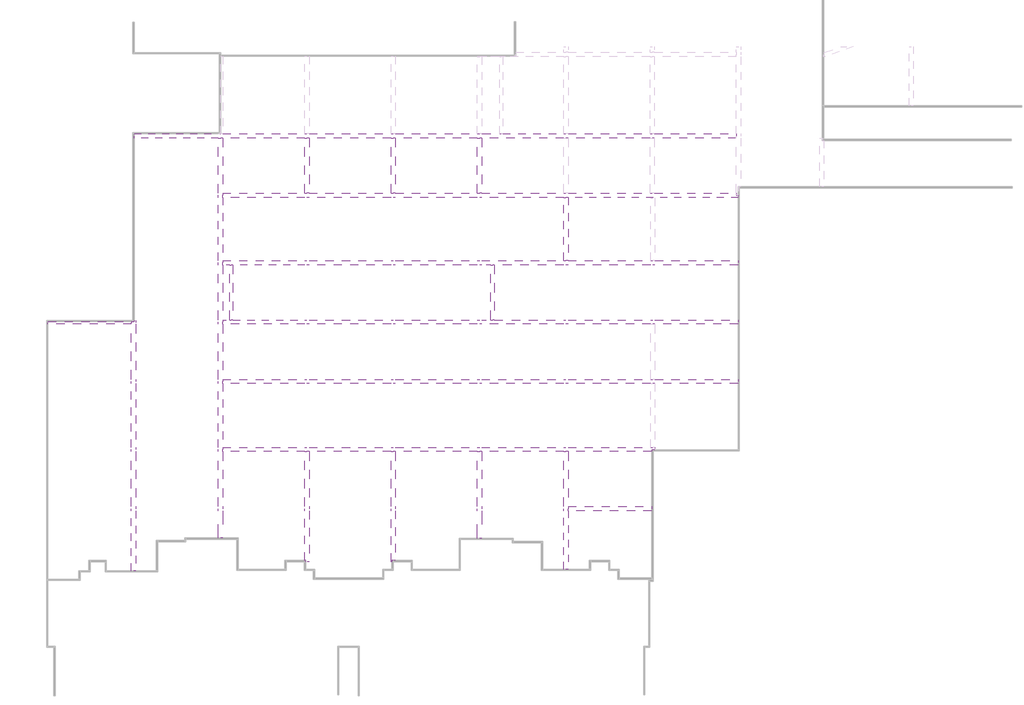
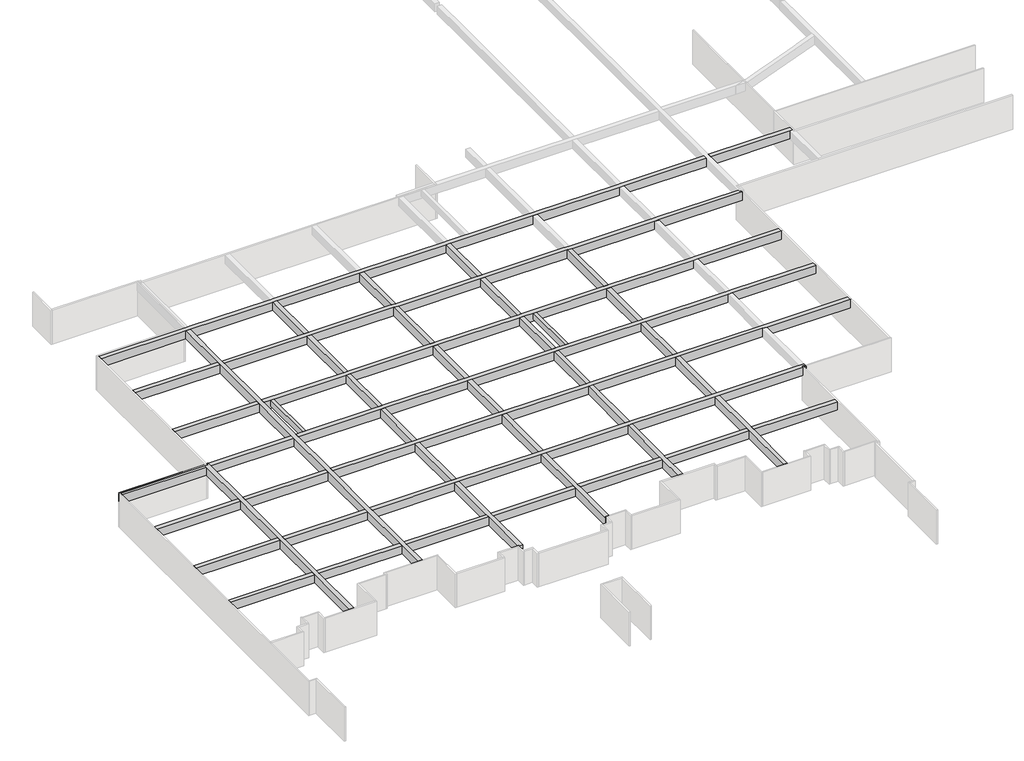
# One storey, part 7 of 14: 20 beams.
"""IFC4 building model written with IfcOpenShell, lengths in millimetres."""

from ifc_helpers import new_model, si_unit, frame, origin, place, context, project, spatial, polyline, outline, extrude, faceted_brep, element, save

model = new_model("IFC4")

# Units and contexts
model_context = context("Model", 3, world=origin())
ifc_project = project(units=[si_unit("LENGTHUNIT", "METRE", prefix="MILLI")], contexts=[model_context])

# Site, building, storey
site = spatial("IfcSite", under=ifc_project)
building = spatial("IfcBuilding", under=site)
storey = spatial("IfcBuildingStorey", under=building, Name="户型图", Elevation=0.0)

# Beams
placement = place(None, origin())
element("IfcBeam", 1, ObjectType="混凝土 - 矩形梁 : KL_beam", at=placement, inside=storey, context=model_context, shape_type="Brep", body=[
    faceted_brep([(-586071.2602569, -192842.8565135, 3300.0), (-586071.2602569, -193242.8565135, 3300.0), (-578267.6529954, -193242.8565135, 3300.0), (-577867.6529954, -193242.8565135, 3300.0), (-570267.6529954, -193242.8565135, 3300.0), (-569867.6529954, -193242.8565135, 3300.0), (-562267.6529954, -193242.8565135, 3300.0), (-561867.6529954, -193242.8565135, 3300.0), (-554267.6529954, -193242.8565135, 3300.0), (-553867.6529954, -193242.8565135, 3300.0), (-546267.6529954, -193242.8565135, 3300.0), (-545867.6529954, -193242.8565135, 3300.0), (-538267.6529954, -193242.8565135, 3300.0), (-537867.6529954, -193242.8565135, 3300.0), (-530267.6529954, -193242.8565135, 3300.0), (-530267.6529954, -192842.8565135, 3300.0), (-537867.6529954, -192842.8565135, 3300.0), (-538267.6529954, -192842.8565135, 3300.0), (-545867.6529954, -192842.8565135, 3300.0), (-546267.6529954, -192842.8565135, 3300.0), (-551917.6529953, -192842.8565135, 3300.0), (-552217.6529953, -192842.8565135, 3300.0), (-553867.6529954, -192842.8565135, 3300.0), (-554267.6529954, -192842.8565135, 3300.0), (-561867.6529954, -192842.8565135, 3300.0), (-562267.6529954, -192842.8565135, 3300.0), (-569867.6529954, -192842.8565135, 3300.0), (-570267.6529954, -192842.8565135, 3300.0), (-577867.6529954, -192842.8565135, 3300.0), (-578267.6529954, -192842.8565135, 3300.0), (-586071.2602569, -193242.8565135, 2500.0), (-578267.6529954, -193242.8565135, 2500.0), (-577867.6529954, -193242.8565135, 2500.0), (-570267.6529954, -193242.8565135, 2500.0), (-569867.6529954, -193242.8565135, 2500.0), (-562267.6529954, -193242.8565135, 2500.0), (-561867.6529954, -193242.8565135, 2500.0), (-554267.6529954, -193242.8565135, 2500.0), (-553867.6529954, -193242.8565135, 2500.0), (-546267.6529954, -193242.8565135, 2500.0), (-545867.6529954, -193242.8565135, 2500.0), (-538267.6529954, -193242.8565135, 2500.0), (-537867.6529954, -193242.8565135, 2500.0), (-530267.6529954, -193242.8565135, 2500.0), (-586071.2602569, -192842.8565135, 2500.0), (-578267.6529954, -192842.8565135, 2500.0), (-577867.6529954, -192842.8565135, 2500.0), (-570267.6529954, -192842.8565135, 2500.0), (-569867.6529954, -192842.8565135, 2500.0), (-562267.6529954, -192842.8565135, 2500.0), (-561867.6529954, -192842.8565135, 2500.0), (-554267.6529954, -192842.8565135, 2500.0), (-553867.6529954, -192842.8565135, 2500.0), (-546267.6529954, -192842.8565135, 2500.0), (-545867.6529954, -192842.8565135, 2500.0), (-538267.6529954, -192842.8565135, 2500.0), (-537867.6529954, -192842.8565135, 2500.0), (-530267.6529954, -192842.8565135, 2500.0)], [[[0, 1, 2, 3, 4, 5, 6, 7, 8, 9, 10, 11, 12, 13, 14, 15, 16, 17, 18, 19, 20, 21, 22, 23, 24, 25, 26, 27, 28, 29]], [[1, 30, 31, 32, 33, 34, 35, 36, 37, 38, 39, 40, 41, 42, 43, 14, 13, 12, 11, 10, 9, 8, 7, 6, 5, 4, 3, 2]], [[30, 44, 45, 46, 47, 48, 49, 50, 51, 52, 53, 54, 55, 56, 57, 43, 42, 41, 40, 39, 38, 37, 36, 35, 34, 33, 32, 31]], [[44, 0, 29, 28, 27, 26, 25, 24, 23, 22, 21, 20, 19, 18, 17, 16, 15, 57, 56, 55, 54, 53, 52, 51, 50, 49, 48, 47, 46, 45]], [[1, 0, 44, 30]], [[15, 14, 43, 57]]]),
    faceted_brep([(-522315.6671501, -192842.8565135, 3300.0), (-522315.6671501, -193242.8565135, 3300.0), (-522315.6671501, -193242.8565135, 2500.0), (-522315.6671501, -192842.8565135, 2500.0), (-529867.6529954, -193242.8565135, 3300.0), (-529867.6529954, -192842.8565135, 3300.0), (-529867.6529954, -192842.8565135, 2500.0), (-529867.6529954, -193242.8565135, 2500.0), (-522567.6529953, -193242.8565135, 3300.0), (-522567.6529953, -193242.8565135, 2500.0)], [[[0, 1, 2, 3]], [[4, 5, 6, 7]], [[1, 0, 5, 4, 8]], [[2, 1, 8, 4, 7, 9]], [[3, 2, 9, 7, 6]], [[0, 3, 6, 5]]]),
])
element("IfcBeam", 2, ObjectType="混凝土 - 矩形梁 : KL_beam", at=placement, inside=storey, context=model_context, shape_type="Brep", body=[
    faceted_brep([(-578267.6529954, -230304.5164481, 3300.0), (-577867.6529954, -230304.5164481, 3300.0), (-577867.6529954, -227792.8565135, 3300.0), (-577867.6529954, -227392.8565135, 3300.0), (-577867.6529954, -222292.8565135, 3300.0), (-577867.6529954, -221892.8565135, 3300.0), (-577867.6529954, -215992.8565135, 3300.0), (-577867.6529954, -215592.8565135, 3300.0), (-577867.6529954, -210492.8565135, 3300.0), (-577867.6529954, -210092.8565135, 3300.0), (-577867.6529954, -204992.8565135, 3300.0), (-577867.6529954, -204592.8565135, 3300.0), (-577867.6529954, -198734.4327531, 3300.0), (-577867.6529954, -198334.4327531, 3300.0), (-577867.6529954, -193242.8565135, 3300.0), (-578267.6529954, -193242.8565135, 3300.0), (-578267.6529954, -198334.4327531, 3300.0), (-578267.6529954, -198734.4327531, 3300.0), (-578267.6529954, -204592.8565135, 3300.0), (-578267.6529954, -204992.8565135, 3300.0), (-578267.6529954, -210092.8565135, 3300.0), (-578267.6529954, -210492.8565135, 3300.0), (-578267.6529954, -215592.8565135, 3300.0), (-578267.6529954, -215992.8565135, 3300.0), (-578267.6529954, -221892.8565135, 3300.0), (-578267.6529954, -222292.8565135, 3300.0), (-578267.6529954, -227392.8565135, 3300.0), (-578267.6529954, -227792.8565135, 3300.0), (-578267.6529954, -230304.5164481, 2500.0), (-578267.6529954, -193242.8565135, 2500.0), (-578267.6529954, -198334.4327531, 2500.0), (-578267.6529954, -198734.4327531, 2500.0), (-578267.6529954, -204592.8565135, 2500.0), (-578267.6529954, -204992.8565135, 2500.0), (-578267.6529954, -210092.8565135, 2500.0), (-578267.6529954, -210492.8565135, 2500.0), (-578267.6529954, -215592.8565135, 2500.0), (-578267.6529954, -215992.8565135, 2500.0), (-578267.6529954, -221892.8565135, 2500.0), (-578267.6529954, -222292.8565135, 2500.0), (-578267.6529954, -227392.8565135, 2500.0), (-578267.6529954, -227792.8565135, 2500.0), (-577867.6529954, -230304.5164481, 2500.0), (-577867.6529954, -193242.8565135, 2500.0), (-577867.6529954, -198334.4327531, 2500.0), (-577867.6529954, -198734.4327531, 2500.0), (-577867.6529954, -204592.8565135, 2500.0), (-577867.6529954, -204992.8565135, 2500.0), (-577867.6529954, -210092.8565135, 2500.0), (-577867.6529954, -210492.8565135, 2500.0), (-577867.6529954, -215592.8565135, 2500.0), (-577867.6529954, -215992.8565135, 2500.0), (-577867.6529954, -221892.8565135, 2500.0), (-577867.6529954, -222292.8565135, 2500.0), (-577867.6529954, -227392.8565135, 2500.0), (-577867.6529954, -227792.8565135, 2500.0)], [[[0, 1, 2, 3, 4, 5, 6, 7, 8, 9, 10, 11, 12, 13, 14, 15, 16, 17, 18, 19, 20, 21, 22, 23, 24, 25, 26, 27]], [[28, 0, 27, 26, 25, 24, 23, 22, 21, 20, 19, 18, 17, 16, 15, 29, 30, 31, 32, 33, 34, 35, 36, 37, 38, 39, 40, 41]], [[42, 28, 41, 40, 39, 38, 37, 36, 35, 34, 33, 32, 31, 30, 29, 43, 44, 45, 46, 47, 48, 49, 50, 51, 52, 53, 54, 55]], [[1, 42, 55, 54, 53, 52, 51, 50, 49, 48, 47, 46, 45, 44, 43, 14, 13, 12, 11, 10, 9, 8, 7, 6, 5, 4, 3, 2]], [[1, 0, 28, 42]], [[15, 14, 43, 29]]]),
])
element("IfcBeam", 3, ObjectType="混凝土 - 矩形梁 : KL_beam", at=placement, inside=storey, context=model_context, shape_type="Brep", body=[
    faceted_brep([(-586071.2602569, -210252.8565135, 3300.0), (-586191.2602569, -210252.8565135, 3300.0), (-586331.2602569, -210252.8565135, 3300.0), (-586331.2602569, -210492.8565135, 3300.0), (-586331.2602569, -215592.8565135, 3300.0), (-586331.2602569, -215992.8565135, 3300.0), (-586331.2602569, -221892.8565135, 3300.0), (-586331.2602569, -222292.8565135, 3300.0), (-586331.2602569, -227392.8565135, 3300.0), (-586331.2602569, -227792.8565135, 3300.0), (-586331.2602569, -233343.599968, 3300.0), (-585931.2602569, -233343.599968, 3300.0), (-585931.2602569, -227792.8565135, 3300.0), (-585931.2602569, -227392.8565135, 3300.0), (-585931.2602569, -222292.8565135, 3300.0), (-585931.2602569, -221892.8565135, 3300.0), (-585931.2602569, -215992.8565135, 3300.0), (-585931.2602569, -215592.8565135, 3300.0), (-585931.2602569, -210492.8565135, 3300.0), (-585931.2602569, -210132.8565135, 3300.0), (-586071.2602569, -210132.8565135, 3300.0), (-586331.2602569, -210252.8565135, 2500.0), (-586331.2602569, -210492.8565135, 2500.0), (-586331.2602569, -215592.8565135, 2500.0), (-586331.2602569, -215992.8565135, 2500.0), (-586331.2602569, -221892.8565135, 2500.0), (-586331.2602569, -222292.8565135, 2500.0), (-586331.2602569, -227392.8565135, 2500.0), (-586331.2602569, -227792.8565135, 2500.0), (-586331.2602569, -233343.599968, 2500.0), (-586071.2602569, -210252.8565135, 2500.0), (-586071.2602569, -210132.8565135, 2500.0), (-585931.2602569, -210132.8565135, 2500.0), (-585931.2602569, -210492.8565135, 2500.0), (-585931.2602569, -215592.8565135, 2500.0), (-585931.2602569, -215992.8565135, 2500.0), (-585931.2602569, -221892.8565135, 2500.0), (-585931.2602569, -222292.8565135, 2500.0), (-585931.2602569, -227392.8565135, 2500.0), (-585931.2602569, -227792.8565135, 2500.0), (-585931.2602569, -233343.599968, 2500.0)], [[[0, 1, 2, 3, 4, 5, 6, 7, 8, 9, 10, 11, 12, 13, 14, 15, 16, 17, 18, 19, 20]], [[2, 21, 22, 23, 24, 25, 26, 27, 28, 29, 10, 9, 8, 7, 6, 5, 4, 3]], [[21, 30, 31, 32, 33, 34, 35, 36, 37, 38, 39, 40, 29, 28, 27, 26, 25, 24, 23, 22]], [[32, 19, 18, 17, 16, 15, 14, 13, 12, 11, 40, 39, 38, 37, 36, 35, 34, 33]], [[19, 32, 31, 20]], [[0, 30, 21, 2, 1]], [[11, 10, 29, 40]], [[30, 0, 20, 31]]]),
])
element("IfcBeam", 4, ObjectType="混凝土 - 矩形梁 : KL_beam", at=placement, inside=storey, context=model_context, shape_type="SweptSolid", body=[
    extrude(outline(polyline([(-594071.2602569, -210492.8565135), (-594071.2602569, -210252.8565135), (-586331.2602569, -210252.8565135), (-586331.2602569, -210492.8565135), (-594071.2602569, -210492.8565135)])), frame((0.0, 0.0, 2500.0), z_axis=(0.0, 0.0, 1.0), x_axis=(1.0, 0.0, 0.0)), (0.0, 0.0, 1.0), 800.0),
    extrude(outline(polyline([(-585931.2602569, -210092.8565135), (-585931.2602569, -210132.8565135), (-586071.2602569, -210132.8565135), (-586071.2602569, -210092.8565135), (-585931.2602569, -210092.8565135)])), frame((0.0, 0.0, 2500.0), z_axis=(0.0, 0.0, 1.0), x_axis=(1.0, 0.0, 0.0)), (0.0, 0.0, 1.0), 800.0),
    extrude(outline(polyline([(-594191.2602569, -210132.8565135), (-594191.2602569, -210092.8565135), (-586191.2602569, -210092.8565135), (-586191.2602569, -210132.8565135), (-594191.2602569, -210132.8565135)])), frame((0.0, 0.0, 2500.0), z_axis=(0.0, 0.0, 1.0), x_axis=(1.0, 0.0, 0.0)), (0.0, 0.0, 1.0), 800.0),
])
element("IfcBeam", 5, ObjectType="混凝土 - 矩形梁 : KL_beam", at=placement, inside=storey, context=model_context, shape_type="Brep", body=[
    faceted_brep([(-585931.2602569, -210092.8565135, 3300.0), (-585931.2602569, -210132.8565135, 3300.0), (-585931.2602569, -210492.8565135, 3300.0), (-578267.6529954, -210492.8565135, 3300.0), (-578267.6529954, -210092.8565135, 3300.0), (-585931.2602569, -210492.8565135, 2500.0), (-578267.6529954, -210492.8565135, 2500.0), (-585931.2602569, -210132.8565135, 2500.0), (-585931.2602569, -210092.8565135, 2500.0), (-578267.6529954, -210092.8565135, 2500.0)], [[[0, 1, 2, 3, 4]], [[2, 5, 6, 3]], [[5, 7, 8, 9, 6]], [[8, 0, 4, 9]], [[5, 2, 1, 0, 8, 7]], [[4, 3, 6, 9]]]),
    faceted_brep([(-530117.7352575, -210092.8565135, 3300.0), (-530117.7352575, -210492.8565135, 3300.0), (-530117.7352575, -210492.8565135, 2500.0), (-530117.7352575, -210092.8565135, 2500.0), (-577867.6529954, -210492.8565135, 3300.0), (-577867.6529954, -210092.8565135, 3300.0), (-577867.6529954, -210092.8565135, 2500.0), (-577867.6529954, -210492.8565135, 2500.0), (-537831.2602569, -210092.8565135, 3300.0), (-538231.2602569, -210092.8565135, 3300.0), (-545867.6529954, -210092.8565135, 3300.0), (-546267.6529954, -210092.8565135, 3300.0), (-552717.6529953, -210092.8565135, 3300.0), (-553017.6529953, -210092.8565135, 3300.0), (-553867.6529954, -210092.8565135, 3300.0), (-554267.6529954, -210092.8565135, 3300.0), (-561867.6529954, -210092.8565135, 3300.0), (-562267.6529954, -210092.8565135, 3300.0), (-569867.6529954, -210092.8565135, 3300.0), (-570267.6529954, -210092.8565135, 3300.0), (-576917.6529953, -210092.8565135, 3300.0), (-577217.6529953, -210092.8565135, 3300.0), (-570267.6529954, -210492.8565135, 3300.0), (-569867.6529954, -210492.8565135, 3300.0), (-562267.6529954, -210492.8565135, 3300.0), (-561867.6529954, -210492.8565135, 3300.0), (-554267.6529954, -210492.8565135, 3300.0), (-553867.6529954, -210492.8565135, 3300.0), (-546267.6529954, -210492.8565135, 3300.0), (-545867.6529954, -210492.8565135, 3300.0), (-538231.2602569, -210492.8565135, 3300.0), (-537831.2602569, -210492.8565135, 3300.0), (-570267.6529954, -210492.8565135, 2500.0), (-569867.6529954, -210492.8565135, 2500.0), (-562267.6529954, -210492.8565135, 2500.0), (-561867.6529954, -210492.8565135, 2500.0), (-554267.6529954, -210492.8565135, 2500.0), (-553867.6529954, -210492.8565135, 2500.0), (-546267.6529954, -210492.8565135, 2500.0), (-545867.6529954, -210492.8565135, 2500.0), (-538231.2602569, -210492.8565135, 2500.0), (-537831.2602569, -210492.8565135, 2500.0), (-570267.6529954, -210092.8565135, 2500.0), (-569867.6529954, -210092.8565135, 2500.0), (-562267.6529954, -210092.8565135, 2500.0), (-561867.6529954, -210092.8565135, 2500.0), (-554267.6529954, -210092.8565135, 2500.0), (-553867.6529954, -210092.8565135, 2500.0), (-546267.6529954, -210092.8565135, 2500.0), (-545867.6529954, -210092.8565135, 2500.0), (-538231.2602569, -210092.8565135, 2500.0), (-537831.2602569, -210092.8565135, 2500.0)], [[[0, 1, 2, 3]], [[4, 5, 6, 7]], [[1, 0, 8, 9, 10, 11, 12, 13, 14, 15, 16, 17, 18, 19, 20, 21, 5, 4, 22, 23, 24, 25, 26, 27, 28, 29, 30, 31]], [[2, 1, 31, 30, 29, 28, 27, 26, 25, 24, 23, 22, 4, 7, 32, 33, 34, 35, 36, 37, 38, 39, 40, 41]], [[3, 2, 41, 40, 39, 38, 37, 36, 35, 34, 33, 32, 7, 6, 42, 43, 44, 45, 46, 47, 48, 49, 50, 51]], [[0, 3, 51, 50, 49, 48, 47, 46, 45, 44, 43, 42, 6, 5, 21, 20, 19, 18, 17, 16, 15, 14, 13, 12, 11, 10, 9, 8]]]),
])
element("IfcBeam", 6, ObjectType="混凝土 - 矩形梁 : KL_beam", at=placement, inside=storey, context=model_context, shape_type="Brep", body=[
    faceted_brep([(-586071.2602569, -204592.8565135, 3300.0), (-586071.2602569, -204992.8565135, 3300.0), (-578267.6529954, -204992.8565135, 3300.0), (-578267.6529954, -204592.8565135, 3300.0), (-586071.2602569, -204992.8565135, 2500.0), (-578267.6529954, -204992.8565135, 2500.0), (-586071.2602569, -204592.8565135, 2500.0), (-578267.6529954, -204592.8565135, 2500.0)], [[[0, 1, 2, 3]], [[1, 4, 5, 2]], [[4, 6, 7, 5]], [[6, 0, 3, 7]], [[1, 0, 6, 4]], [[3, 2, 5, 7]]]),
    faceted_brep([(-530117.7352575, -204592.8565135, 3300.0), (-530117.7352575, -204992.8565135, 3300.0), (-530117.7352575, -204992.8565135, 2500.0), (-530117.7352575, -204592.8565135, 2500.0), (-577867.6529954, -204992.8565135, 3300.0), (-577867.6529954, -204592.8565135, 3300.0), (-577867.6529954, -204592.8565135, 2500.0), (-577867.6529954, -204992.8565135, 2500.0), (-537831.2602569, -204592.8565135, 3300.0), (-538231.2602569, -204592.8565135, 3300.0), (-545867.6529954, -204592.8565135, 3300.0), (-546267.6529954, -204592.8565135, 3300.0), (-553867.6529954, -204592.8565135, 3300.0), (-554267.6529954, -204592.8565135, 3300.0), (-561867.6529954, -204592.8565135, 3300.0), (-562267.6529954, -204592.8565135, 3300.0), (-569867.6529954, -204592.8565135, 3300.0), (-570267.6529954, -204592.8565135, 3300.0), (-577217.6529953, -204992.8565135, 3300.0), (-576917.6529953, -204992.8565135, 3300.0), (-570267.6529954, -204992.8565135, 3300.0), (-569867.6529954, -204992.8565135, 3300.0), (-562267.6529954, -204992.8565135, 3300.0), (-561867.6529954, -204992.8565135, 3300.0), (-554267.6529954, -204992.8565135, 3300.0), (-553867.6529954, -204992.8565135, 3300.0), (-553017.6529953, -204992.8565135, 3300.0), (-552717.6529953, -204992.8565135, 3300.0), (-546267.6529954, -204992.8565135, 3300.0), (-545867.6529954, -204992.8565135, 3300.0), (-538231.2602569, -204992.8565135, 3300.0), (-537831.2602569, -204992.8565135, 3300.0), (-570267.6529954, -204992.8565135, 2500.0), (-569867.6529954, -204992.8565135, 2500.0), (-562267.6529954, -204992.8565135, 2500.0), (-561867.6529954, -204992.8565135, 2500.0), (-554267.6529954, -204992.8565135, 2500.0), (-553867.6529954, -204992.8565135, 2500.0), (-546267.6529954, -204992.8565135, 2500.0), (-545867.6529954, -204992.8565135, 2500.0), (-538231.2602569, -204992.8565135, 2500.0), (-537831.2602569, -204992.8565135, 2500.0), (-570267.6529954, -204592.8565135, 2500.0), (-569867.6529954, -204592.8565135, 2500.0), (-562267.6529954, -204592.8565135, 2500.0), (-561867.6529954, -204592.8565135, 2500.0), (-554267.6529954, -204592.8565135, 2500.0), (-553867.6529954, -204592.8565135, 2500.0), (-546267.6529954, -204592.8565135, 2500.0), (-545867.6529954, -204592.8565135, 2500.0), (-538231.2602569, -204592.8565135, 2500.0), (-537831.2602569, -204592.8565135, 2500.0)], [[[0, 1, 2, 3]], [[4, 5, 6, 7]], [[1, 0, 8, 9, 10, 11, 12, 13, 14, 15, 16, 17, 5, 4, 18, 19, 20, 21, 22, 23, 24, 25, 26, 27, 28, 29, 30, 31]], [[2, 1, 31, 30, 29, 28, 27, 26, 25, 24, 23, 22, 21, 20, 19, 18, 4, 7, 32, 33, 34, 35, 36, 37, 38, 39, 40, 41]], [[3, 2, 41, 40, 39, 38, 37, 36, 35, 34, 33, 32, 7, 6, 42, 43, 44, 45, 46, 47, 48, 49, 50, 51]], [[0, 3, 51, 50, 49, 48, 47, 46, 45, 44, 43, 42, 6, 5, 17, 16, 15, 14, 13, 12, 11, 10, 9, 8]]]),
])
element("IfcBeam", 7, ObjectType="混凝土 - 矩形梁 : KL_beam", at=placement, inside=storey, context=model_context, shape_type="Brep", body=[
    faceted_brep([(-530117.7352575, -198734.4327531, 3300.0), (-530117.7352575, -198534.4327531, 3300.0), (-530267.6529954, -198534.4327531, 3300.0), (-530267.6529954, -198334.4327531, 3300.0), (-537867.6529954, -198334.4327531, 3300.0), (-538267.6529954, -198334.4327531, 3300.0), (-545867.6529954, -198334.4327531, 3300.0), (-546267.6529954, -198334.4327531, 3300.0), (-553867.6529954, -198334.4327531, 3300.0), (-554267.6529954, -198334.4327531, 3300.0), (-561867.6529954, -198334.4327531, 3300.0), (-562267.6529954, -198334.4327531, 3300.0), (-569867.6529954, -198334.4327531, 3300.0), (-570267.6529954, -198334.4327531, 3300.0), (-577867.6529954, -198334.4327531, 3300.0), (-577867.6529954, -198734.4327531, 3300.0), (-570267.6529954, -198734.4327531, 3300.0), (-569867.6529954, -198734.4327531, 3300.0), (-562267.6529954, -198734.4327531, 3300.0), (-561867.6529954, -198734.4327531, 3300.0), (-554267.6529954, -198734.4327531, 3300.0), (-553867.6529954, -198734.4327531, 3300.0), (-546267.6529954, -198734.4327531, 3300.0), (-545867.6529954, -198734.4327531, 3300.0), (-530267.6529954, -198334.4327531, 2500.0), (-537867.6529954, -198334.4327531, 2500.0), (-538267.6529954, -198334.4327531, 2500.0), (-545867.6529954, -198334.4327531, 2500.0), (-546267.6529954, -198334.4327531, 2500.0), (-553867.6529954, -198334.4327531, 2500.0), (-554267.6529954, -198334.4327531, 2500.0), (-561867.6529954, -198334.4327531, 2500.0), (-562267.6529954, -198334.4327531, 2500.0), (-569867.6529954, -198334.4327531, 2500.0), (-570267.6529954, -198334.4327531, 2500.0), (-577867.6529954, -198334.4327531, 2500.0), (-530117.7352575, -198534.4327531, 2500.0), (-530117.7352575, -198734.4327531, 2500.0), (-545867.6529954, -198734.4327531, 2500.0), (-546267.6529954, -198734.4327531, 2500.0), (-553867.6529954, -198734.4327531, 2500.0), (-554267.6529954, -198734.4327531, 2500.0), (-561867.6529954, -198734.4327531, 2500.0), (-562267.6529954, -198734.4327531, 2500.0), (-569867.6529954, -198734.4327531, 2500.0), (-570267.6529954, -198734.4327531, 2500.0), (-577867.6529954, -198734.4327531, 2500.0), (-530267.6529954, -198534.4327531, 2500.0)], [[[0, 1, 2, 3, 4, 5, 6, 7, 8, 9, 10, 11, 12, 13, 14, 15, 16, 17, 18, 19, 20, 21, 22, 23]], [[3, 24, 25, 26, 27, 28, 29, 30, 31, 32, 33, 34, 35, 14, 13, 12, 11, 10, 9, 8, 7, 6, 5, 4]], [[36, 37, 38, 39, 40, 41, 42, 43, 44, 45, 46, 35, 34, 33, 32, 31, 30, 29, 28, 27, 26, 25, 24, 47]], [[37, 0, 23, 22, 21, 20, 19, 18, 17, 16, 15, 46, 45, 44, 43, 42, 41, 40, 39, 38]], [[0, 37, 36, 1]], [[47, 2, 1, 36]], [[2, 47, 24, 3]], [[15, 14, 35, 46]]]),
    faceted_brep([(-586071.2602569, -198734.4327531, 3300.0), (-586071.2602569, -198334.4327531, 3300.0), (-586071.2602569, -198334.4327531, 2500.0), (-586071.2602569, -198734.4327531, 2500.0), (-578267.6529954, -198334.4327531, 3300.0), (-578267.6529954, -198734.4327531, 3300.0), (-578267.6529954, -198734.4327531, 2500.0), (-578267.6529954, -198334.4327531, 2500.0)], [[[0, 1, 2, 3]], [[4, 5, 6, 7]], [[1, 0, 5, 4]], [[2, 1, 4, 7]], [[3, 2, 7, 6]], [[0, 3, 6, 5]]]),
])
element("IfcBeam", 8, ObjectType="混凝土 - 矩形梁 : KL_beam", at=placement, inside=storey, context=model_context, shape_type="SweptSolid", body=[
    extrude(outline(polyline([(-570267.6529954, -193242.8565135), (-569867.6529954, -193242.8565135), (-569867.6529954, -198334.4327531), (-570267.6529954, -198334.4327531), (-570267.6529954, -193242.8565135)])), frame((0.0, 0.0, 2500.0), z_axis=(0.0, 0.0, 1.0), x_axis=(1.0, 0.0, 0.0)), (0.0, 0.0, 1.0), 800.0),
])
element("IfcBeam", 9, ObjectType="混凝土 - 矩形梁 : KL_beam", at=placement, inside=storey, context=model_context, shape_type="SweptSolid", body=[
    extrude(outline(polyline([(-562267.6529954, -193242.8565135), (-561867.6529954, -193242.8565135), (-561867.6529954, -198334.4327531), (-562267.6529954, -198334.4327531), (-562267.6529954, -193242.8565135)])), frame((0.0, 0.0, 2500.0), z_axis=(0.0, 0.0, 1.0), x_axis=(1.0, 0.0, 0.0)), (0.0, 0.0, 1.0), 800.0),
])
element("IfcBeam", 10, ObjectType="混凝土 - 矩形梁 : KL_beam", at=placement, inside=storey, context=model_context, shape_type="SweptSolid", body=[
    extrude(outline(polyline([(-554267.6529954, -193242.8565135), (-553867.6529954, -193242.8565135), (-553867.6529954, -198334.4327531), (-554267.6529954, -198334.4327531), (-554267.6529954, -193242.8565135)])), frame((0.0, 0.0, 2500.0), z_axis=(0.0, 0.0, 1.0), x_axis=(1.0, 0.0, 0.0)), (0.0, 0.0, 1.0), 800.0),
])
element("IfcBeam", 11, ObjectType="混凝土 - 矩形梁 : KL_beam", at=placement, inside=storey, context=model_context, shape_type="Brep", body=[
    faceted_brep([(-530117.7352575, -215992.8565135, 3300.0), (-530117.7352575, -215592.8565135, 3300.0), (-537831.2602569, -215592.8565135, 3300.0), (-538231.2602569, -215592.8565135, 3300.0), (-545867.6529954, -215592.8565135, 3300.0), (-546267.6529954, -215592.8565135, 3300.0), (-553867.6529954, -215592.8565135, 3300.0), (-554267.6529954, -215592.8565135, 3300.0), (-561867.6529954, -215592.8565135, 3300.0), (-562267.6529954, -215592.8565135, 3300.0), (-569867.6529954, -215592.8565135, 3300.0), (-570267.6529954, -215592.8565135, 3300.0), (-577867.6529954, -215592.8565135, 3300.0), (-577867.6529954, -215992.8565135, 3300.0), (-570267.6529954, -215992.8565135, 3300.0), (-569867.6529954, -215992.8565135, 3300.0), (-562267.6529954, -215992.8565135, 3300.0), (-561867.6529954, -215992.8565135, 3300.0), (-554267.6529954, -215992.8565135, 3300.0), (-553867.6529954, -215992.8565135, 3300.0), (-546267.6529954, -215992.8565135, 3300.0), (-545867.6529954, -215992.8565135, 3300.0), (-538231.2602569, -215992.8565135, 3300.0), (-537831.2602569, -215992.8565135, 3300.0), (-530117.7352575, -215592.8565135, 2500.0), (-537831.2602569, -215592.8565135, 2500.0), (-538231.2602569, -215592.8565135, 2500.0), (-545867.6529954, -215592.8565135, 2500.0), (-546267.6529954, -215592.8565135, 2500.0), (-553867.6529954, -215592.8565135, 2500.0), (-554267.6529954, -215592.8565135, 2500.0), (-561867.6529954, -215592.8565135, 2500.0), (-562267.6529954, -215592.8565135, 2500.0), (-569867.6529954, -215592.8565135, 2500.0), (-570267.6529954, -215592.8565135, 2500.0), (-577867.6529954, -215592.8565135, 2500.0), (-530117.7352575, -215992.8565135, 2500.0), (-537831.2602569, -215992.8565135, 2500.0), (-538231.2602569, -215992.8565135, 2500.0), (-545867.6529954, -215992.8565135, 2500.0), (-546267.6529954, -215992.8565135, 2500.0), (-553867.6529954, -215992.8565135, 2500.0), (-554267.6529954, -215992.8565135, 2500.0), (-561867.6529954, -215992.8565135, 2500.0), (-562267.6529954, -215992.8565135, 2500.0), (-569867.6529954, -215992.8565135, 2500.0), (-570267.6529954, -215992.8565135, 2500.0), (-577867.6529954, -215992.8565135, 2500.0)], [[[0, 1, 2, 3, 4, 5, 6, 7, 8, 9, 10, 11, 12, 13, 14, 15, 16, 17, 18, 19, 20, 21, 22, 23]], [[1, 24, 25, 26, 27, 28, 29, 30, 31, 32, 33, 34, 35, 12, 11, 10, 9, 8, 7, 6, 5, 4, 3, 2]], [[24, 36, 37, 38, 39, 40, 41, 42, 43, 44, 45, 46, 47, 35, 34, 33, 32, 31, 30, 29, 28, 27, 26, 25]], [[36, 0, 23, 22, 21, 20, 19, 18, 17, 16, 15, 14, 13, 47, 46, 45, 44, 43, 42, 41, 40, 39, 38, 37]], [[1, 0, 36, 24]], [[13, 12, 35, 47]]]),
    faceted_brep([(-594071.2602569, -215992.8565135, 3300.0), (-594071.2602569, -215592.8565135, 3300.0), (-594071.2602569, -215592.8565135, 2500.0), (-594071.2602569, -215992.8565135, 2500.0), (-586331.2602569, -215992.8565135, 3300.0), (-586331.2602569, -215592.8565135, 3300.0), (-586331.2602569, -215592.8565135, 2500.0), (-586331.2602569, -215992.8565135, 2500.0)], [[[0, 1, 2, 3]], [[1, 0, 4, 5]], [[2, 1, 5, 6]], [[3, 2, 6, 7]], [[0, 3, 7, 4]], [[5, 4, 7, 6]]]),
    faceted_brep([(-578267.6529954, -215592.8565135, 3300.0), (-578267.6529954, -215992.8565135, 3300.0), (-578267.6529954, -215992.8565135, 2500.0), (-578267.6529954, -215592.8565135, 2500.0), (-585931.2602569, -215992.8565135, 3300.0), (-585931.2602569, -215592.8565135, 3300.0), (-585931.2602569, -215592.8565135, 2500.0), (-585931.2602569, -215992.8565135, 2500.0)], [[[0, 1, 2, 3]], [[4, 5, 6, 7]], [[1, 0, 5, 4]], [[0, 3, 6, 5]], [[3, 2, 7, 6]], [[2, 1, 4, 7]]]),
])
element("IfcBeam", 12, ObjectType="混凝土 - 矩形梁 : KL_beam", at=placement, inside=storey, context=model_context, shape_type="Brep", body=[
    faceted_brep([(-594071.2602569, -221892.8565135, 3300.0), (-594071.2602569, -222292.8565135, 3300.0), (-586331.2602569, -222292.8565135, 3300.0), (-586331.2602569, -221892.8565135, 3300.0), (-594071.2602569, -222292.8565135, 2500.0), (-586331.2602569, -222292.8565135, 2500.0), (-594071.2602569, -221892.8565135, 2500.0), (-586331.2602569, -221892.8565135, 2500.0)], [[[0, 1, 2, 3]], [[1, 4, 5, 2]], [[4, 6, 7, 5]], [[6, 0, 3, 7]], [[1, 0, 6, 4]], [[3, 2, 5, 7]]]),
    faceted_brep([(-578267.6529954, -221892.8565135, 3300.0), (-578267.6529954, -222292.8565135, 3300.0), (-578267.6529954, -222292.8565135, 2500.0), (-578267.6529954, -221892.8565135, 2500.0), (-585931.2602569, -222292.8565135, 3300.0), (-585931.2602569, -221892.8565135, 3300.0), (-585931.2602569, -221892.8565135, 2500.0), (-585931.2602569, -222292.8565135, 2500.0)], [[[0, 1, 2, 3]], [[4, 5, 6, 7]], [[1, 0, 5, 4]], [[2, 1, 4, 7]], [[3, 2, 7, 6]], [[0, 3, 6, 5]]]),
    faceted_brep([(-577867.6529954, -222292.8565135, 3300.0), (-577867.6529954, -221892.8565135, 3300.0), (-577867.6529954, -221892.8565135, 2500.0), (-577867.6529954, -222292.8565135, 2500.0), (-570267.6529954, -221892.8565135, 3300.0), (-569867.6529954, -221892.8565135, 3300.0), (-562267.6529954, -221892.8565135, 3300.0), (-561867.6529954, -221892.8565135, 3300.0), (-554267.6529954, -221892.8565135, 3300.0), (-553867.6529954, -221892.8565135, 3300.0), (-546267.6529954, -221892.8565135, 3300.0), (-545867.6529954, -221892.8565135, 3300.0), (-538231.2602569, -221892.8565135, 3300.0), (-537831.2602569, -221892.8565135, 3300.0), (-537831.2602569, -221892.8565135, 2500.0), (-538231.2602569, -221892.8565135, 2500.0), (-545867.6529954, -221892.8565135, 2500.0), (-546267.6529954, -221892.8565135, 2500.0), (-553867.6529954, -221892.8565135, 2500.0), (-554267.6529954, -221892.8565135, 2500.0), (-561867.6529954, -221892.8565135, 2500.0), (-562267.6529954, -221892.8565135, 2500.0), (-569867.6529954, -221892.8565135, 2500.0), (-570267.6529954, -221892.8565135, 2500.0), (-538117.7352575, -222130.9174567, 2500.0), (-538117.7352575, -222130.9174567, 3300.0), (-538117.7352575, -222292.8565135, 3300.0), (-538117.7352575, -222292.8565135, 2500.0), (-537831.2602569, -222130.9174567, 2500.0), (-537831.2602569, -222130.9174567, 3300.0), (-537997.7352575, -222130.9174567, 3300.0), (-570267.6529954, -222292.8565135, 2500.0), (-569867.6529954, -222292.8565135, 2500.0), (-562267.6529954, -222292.8565135, 2500.0), (-561867.6529954, -222292.8565135, 2500.0), (-554267.6529954, -222292.8565135, 2500.0), (-553867.6529954, -222292.8565135, 2500.0), (-546267.6529954, -222292.8565135, 2500.0), (-545867.6529954, -222292.8565135, 2500.0), (-545867.6529954, -222292.8565135, 3300.0), (-546267.6529954, -222292.8565135, 3300.0), (-553867.6529954, -222292.8565135, 3300.0), (-554267.6529954, -222292.8565135, 3300.0), (-561867.6529954, -222292.8565135, 3300.0), (-562267.6529954, -222292.8565135, 3300.0), (-569867.6529954, -222292.8565135, 3300.0), (-570267.6529954, -222292.8565135, 3300.0)], [[[0, 1, 2, 3]], [[2, 1, 4, 5, 6, 7, 8, 9, 10, 11, 12, 13, 14, 15, 16, 17, 18, 19, 20, 21, 22, 23]], [[24, 25, 26, 27]], [[25, 24, 28, 29, 30]], [[0, 3, 31, 32, 33, 34, 35, 36, 37, 38, 27, 26, 39, 40, 41, 42, 43, 44, 45, 46]], [[1, 0, 46, 45, 44, 43, 42, 41, 40, 39, 26, 25, 30, 29, 13, 12, 11, 10, 9, 8, 7, 6, 5, 4]], [[3, 2, 23, 22, 21, 20, 19, 18, 17, 16, 15, 14, 28, 24, 27, 38, 37, 36, 35, 34, 33, 32, 31]], [[14, 13, 29, 28]]]),
    faceted_brep([(-537997.7352575, -222292.8565135, 3300.0), (-537831.2602569, -222292.8565135, 3300.0), (-537831.2602569, -222250.9174567, 3300.0), (-537997.7352575, -222250.9174567, 3300.0), (-537831.2602569, -222292.8565135, 2500.0), (-537997.7352575, -222292.8565135, 2500.0), (-537997.7352575, -222250.9174567, 2500.0), (-537831.2602569, -222250.9174567, 2500.0)], [[[0, 1, 2, 3]], [[4, 1, 0, 5]], [[4, 5, 6, 7]], [[1, 4, 7, 2]], [[5, 0, 3, 6]], [[3, 2, 7, 6]]]),
])
element("IfcBeam", 13, ObjectType="混凝土 - 矩形梁 : KL_beam", at=placement, inside=storey, context=model_context, shape_type="Brep", body=[
    faceted_brep([(-545867.6529954, -204992.8565135, 3300.0), (-546267.6529954, -204992.8565135, 3300.0), (-546267.6529954, -210092.8565135, 3300.0), (-545867.6529954, -210092.8565135, 3300.0), (-546267.6529954, -204992.8565135, 2500.0), (-546267.6529954, -210092.8565135, 2500.0), (-545867.6529954, -204992.8565135, 2500.0), (-545867.6529954, -210092.8565135, 2500.0)], [[[0, 1, 2, 3]], [[1, 4, 5, 2]], [[4, 6, 7, 5]], [[6, 0, 3, 7]], [[1, 0, 6, 4]], [[3, 2, 5, 7]]]),
    faceted_brep([(-545867.6529954, -233209.9306648, 3300.0), (-546267.6529954, -233209.9306648, 3300.0), (-546267.6529954, -233209.9306648, 2500.0), (-545867.6529954, -233209.9306648, 2500.0), (-546267.6529954, -222292.8565135, 3300.0), (-545867.6529954, -222292.8565135, 3300.0), (-545867.6529954, -222292.8565135, 2500.0), (-546267.6529954, -222292.8565135, 2500.0), (-545867.6529954, -227792.8565135, 3300.0), (-545867.6529954, -227392.8565135, 3300.0), (-546267.6529954, -227392.8565135, 3300.0), (-546267.6529954, -227792.8565135, 3300.0), (-546267.6529954, -227392.8565135, 2500.0), (-546267.6529954, -227792.8565135, 2500.0), (-545867.6529954, -227392.8565135, 2500.0), (-545867.6529954, -227792.8565135, 2500.0)], [[[0, 1, 2, 3]], [[4, 5, 6, 7]], [[1, 0, 8, 9, 5, 4, 10, 11]], [[2, 1, 11, 10, 4, 7, 12, 13]], [[3, 2, 13, 12, 7, 6, 14, 15]], [[0, 3, 15, 14, 6, 5, 9, 8]]]),
    faceted_brep([(-546267.6529954, -210492.8565135, 3300.0), (-545867.6529954, -210492.8565135, 3300.0), (-545867.6529954, -210492.8565135, 2500.0), (-546267.6529954, -210492.8565135, 2500.0), (-545867.6529954, -215592.8565135, 3300.0), (-546267.6529954, -215592.8565135, 3300.0), (-546267.6529954, -215592.8565135, 2500.0), (-545867.6529954, -215592.8565135, 2500.0)], [[[0, 1, 2, 3]], [[4, 5, 6, 7]], [[1, 0, 5, 4]], [[0, 3, 6, 5]], [[3, 2, 7, 6]], [[2, 1, 4, 7]]]),
    faceted_brep([(-545867.6529954, -215992.8565135, 3300.0), (-546267.6529954, -215992.8565135, 3300.0), (-546267.6529954, -221892.8565135, 3300.0), (-545867.6529954, -221892.8565135, 3300.0), (-546267.6529954, -215992.8565135, 2500.0), (-546267.6529954, -221892.8565135, 2500.0), (-545867.6529954, -215992.8565135, 2500.0), (-545867.6529954, -221892.8565135, 2500.0)], [[[0, 1, 2, 3]], [[1, 4, 5, 2]], [[4, 6, 7, 5]], [[6, 0, 3, 7]], [[1, 0, 6, 4]], [[3, 2, 5, 7]]]),
])
element("IfcBeam", 14, ObjectType="混凝土 - 矩形梁 : KL_beam", at=placement, inside=storey, context=model_context, shape_type="Brep", body=[
    faceted_brep([(-554267.6529954, -230332.9126843, 3300.0), (-553867.6529954, -230332.9126843, 3300.0), (-553867.6529954, -227792.8565135, 3300.0), (-553867.6529954, -227392.8565135, 3300.0), (-553867.6529954, -222292.8565135, 3300.0), (-554267.6529954, -222292.8565135, 3300.0), (-554267.6529954, -227392.8565135, 3300.0), (-554267.6529954, -227792.8565135, 3300.0), (-553867.6529954, -230332.9126843, 2500.0), (-553867.6529954, -227792.8565135, 2500.0), (-553867.6529954, -227392.8565135, 2500.0), (-553867.6529954, -222292.8565135, 2500.0), (-554267.6529954, -230332.9126843, 2500.0), (-554267.6529954, -227792.8565135, 2500.0), (-554267.6529954, -227392.8565135, 2500.0), (-554267.6529954, -222292.8565135, 2500.0)], [[[0, 1, 2, 3, 4, 5, 6, 7]], [[1, 8, 9, 10, 11, 4, 3, 2]], [[8, 12, 13, 14, 15, 11, 10, 9]], [[12, 0, 7, 6, 5, 15, 14, 13]], [[1, 0, 12, 8]], [[5, 4, 11, 15]]]),
    faceted_brep([(-554267.6529954, -198734.4327531, 3300.0), (-553867.6529954, -198734.4327531, 3300.0), (-553867.6529954, -198734.4327531, 2500.0), (-554267.6529954, -198734.4327531, 2500.0), (-554267.6529954, -204592.8565135, 3300.0), (-553867.6529954, -204592.8565135, 3300.0), (-553867.6529954, -204592.8565135, 2500.0), (-554267.6529954, -204592.8565135, 2500.0)], [[[0, 1, 2, 3]], [[1, 0, 4, 5]], [[2, 1, 5, 6]], [[3, 2, 6, 7]], [[0, 3, 7, 4]], [[5, 4, 7, 6]]]),
    faceted_brep([(-554267.6529954, -210492.8565135, 3300.0), (-553867.6529954, -210492.8565135, 3300.0), (-553867.6529954, -210492.8565135, 2500.0), (-554267.6529954, -210492.8565135, 2500.0), (-553867.6529954, -215592.8565135, 3300.0), (-554267.6529954, -215592.8565135, 3300.0), (-554267.6529954, -215592.8565135, 2500.0), (-553867.6529954, -215592.8565135, 2500.0)], [[[0, 1, 2, 3]], [[4, 5, 6, 7]], [[1, 0, 5, 4]], [[2, 1, 4, 7]], [[3, 2, 7, 6]], [[0, 3, 6, 5]]]),
    faceted_brep([(-553867.6529954, -210092.8565135, 3300.0), (-554267.6529954, -210092.8565135, 3300.0), (-554267.6529954, -210092.8565135, 2500.0), (-553867.6529954, -210092.8565135, 2500.0), (-554267.6529954, -204992.8565135, 3300.0), (-553867.6529954, -204992.8565135, 3300.0), (-553867.6529954, -204992.8565135, 2500.0), (-554267.6529954, -204992.8565135, 2500.0)], [[[0, 1, 2, 3]], [[4, 5, 6, 7]], [[1, 0, 5, 4]], [[0, 3, 6, 5]], [[3, 2, 7, 6]], [[2, 1, 4, 7]]]),
    faceted_brep([(-554267.6529954, -215992.8565135, 3300.0), (-553867.6529954, -215992.8565135, 3300.0), (-553867.6529954, -215992.8565135, 2500.0), (-554267.6529954, -215992.8565135, 2500.0), (-553867.6529954, -221892.8565135, 3300.0), (-554267.6529954, -221892.8565135, 3300.0), (-554267.6529954, -221892.8565135, 2500.0), (-553867.6529954, -221892.8565135, 2500.0)], [[[0, 1, 2, 3]], [[4, 5, 6, 7]], [[1, 0, 5, 4]], [[2, 1, 4, 7]], [[3, 2, 7, 6]], [[0, 3, 6, 5]]]),
])
element("IfcBeam", 15, ObjectType="混凝土 - 矩形梁 : KL_beam", at=placement, inside=storey, context=model_context, shape_type="SweptSolid", body=[
    extrude(outline(polyline([(-545867.6529954, -204592.8565135), (-546267.6529954, -204592.8565135), (-546267.6529954, -198734.4327531), (-545867.6529954, -198734.4327531), (-545867.6529954, -204592.8565135)])), frame((0.0, 0.0, 2500.0), z_axis=(0.0, 0.0, 1.0), x_axis=(1.0, 0.0, 0.0)), (0.0, 0.0, 1.0), 800.0),
])
element("IfcBeam", 16, ObjectType="混凝土 - 矩形梁 : KL_beam", at=placement, inside=storey, context=model_context, shape_type="Brep", body=[
    faceted_brep([(-561867.6529954, -198734.4327531, 3300.0), (-562267.6529954, -198734.4327531, 3300.0), (-562267.6529954, -204592.8565135, 3300.0), (-561867.6529954, -204592.8565135, 3300.0), (-562267.6529954, -198734.4327531, 2500.0), (-562267.6529954, -204592.8565135, 2500.0), (-561867.6529954, -198734.4327531, 2500.0), (-561867.6529954, -204592.8565135, 2500.0)], [[[0, 1, 2, 3]], [[1, 4, 5, 2]], [[4, 6, 7, 5]], [[6, 0, 3, 7]], [[1, 0, 6, 4]], [[3, 2, 5, 7]]]),
    faceted_brep([(-562267.6529954, -232514.6386108, 3300.0), (-562267.6529954, -232514.6386108, 2500.0), (-562209.7925406, -232514.6386108, 2500.0), (-562209.7925406, -232514.6386108, 3300.0), (-562209.7925406, -232394.6386108, 3300.0), (-562209.7925406, -232394.6386108, 2500.0), (-561867.6529954, -232394.6386108, 2500.0), (-561867.6529954, -232394.6386108, 3300.0), (-562089.7925406, -232394.6386108, 3300.0), (-562267.6529954, -222292.8565135, 3300.0), (-561867.6529954, -222292.8565135, 3300.0), (-561867.6529954, -222292.8565135, 2500.0), (-562267.6529954, -222292.8565135, 2500.0), (-561867.6529954, -227792.8565135, 3300.0), (-561867.6529954, -227392.8565135, 3300.0), (-562267.6529954, -227392.8565135, 3300.0), (-562267.6529954, -227792.8565135, 3300.0), (-562267.6529954, -227392.8565135, 2500.0), (-562267.6529954, -227792.8565135, 2500.0), (-561867.6529954, -227392.8565135, 2500.0), (-561867.6529954, -227792.8565135, 2500.0)], [[[0, 1, 2, 3]], [[4, 5, 6, 7, 8]], [[9, 10, 11, 12]], [[4, 8, 7, 13, 14, 10, 9, 15, 16, 0, 3]], [[1, 0, 16, 15, 9, 12, 17, 18]], [[6, 5, 2, 1, 18, 17, 12, 11, 19, 20]], [[7, 6, 20, 19, 11, 10, 14, 13]], [[5, 4, 3, 2]]]),
    faceted_brep([(-562267.6529954, -210492.8565135, 3300.0), (-561867.6529954, -210492.8565135, 3300.0), (-561867.6529954, -210492.8565135, 2500.0), (-562267.6529954, -210492.8565135, 2500.0), (-561867.6529954, -215592.8565135, 3300.0), (-562267.6529954, -215592.8565135, 3300.0), (-562267.6529954, -215592.8565135, 2500.0), (-561867.6529954, -215592.8565135, 2500.0)], [[[0, 1, 2, 3]], [[4, 5, 6, 7]], [[1, 0, 5, 4]], [[0, 3, 6, 5]], [[3, 2, 7, 6]], [[2, 1, 4, 7]]]),
    faceted_brep([(-561867.6529954, -210092.8565135, 3300.0), (-562267.6529954, -210092.8565135, 3300.0), (-562267.6529954, -210092.8565135, 2500.0), (-561867.6529954, -210092.8565135, 2500.0), (-562267.6529954, -204992.8565135, 3300.0), (-561867.6529954, -204992.8565135, 3300.0), (-561867.6529954, -204992.8565135, 2500.0), (-562267.6529954, -204992.8565135, 2500.0)], [[[0, 1, 2, 3]], [[4, 5, 6, 7]], [[1, 0, 5, 4]], [[2, 1, 4, 7]], [[3, 2, 7, 6]], [[0, 3, 6, 5]]]),
    faceted_brep([(-561867.6529954, -215992.8565135, 3300.0), (-562267.6529954, -215992.8565135, 3300.0), (-562267.6529954, -221892.8565135, 3300.0), (-561867.6529954, -221892.8565135, 3300.0), (-562267.6529954, -215992.8565135, 2500.0), (-562267.6529954, -221892.8565135, 2500.0), (-561867.6529954, -215992.8565135, 2500.0), (-561867.6529954, -221892.8565135, 2500.0)], [[[0, 1, 2, 3]], [[1, 4, 5, 2]], [[4, 6, 7, 5]], [[6, 0, 3, 7]], [[1, 0, 6, 4]], [[3, 2, 5, 7]]]),
])
element("IfcBeam", 17, ObjectType="混凝土 - 矩形梁 : KL_beam", at=placement, inside=storey, context=model_context, shape_type="Brep", body=[
    faceted_brep([(-569867.6529954, -232514.535682, 2500.0), (-569867.6529954, -232514.535682, 3300.0), (-570188.8878112, -232514.535682, 3300.0), (-570188.8878112, -232514.535682, 2500.0), (-570267.6529954, -222292.8565135, 3300.0), (-569867.6529954, -222292.8565135, 3300.0), (-569867.6529954, -222292.8565135, 2500.0), (-570267.6529954, -222292.8565135, 2500.0), (-569867.6529954, -227792.8565135, 3300.0), (-569867.6529954, -227392.8565135, 3300.0), (-570267.6529954, -227392.8565135, 3300.0), (-570267.6529954, -227792.8565135, 3300.0), (-570267.6529954, -232394.6386108, 3300.0), (-570188.8878112, -232394.6386108, 3300.0), (-569867.6529954, -227792.8565135, 2500.0), (-569867.6529954, -227392.8565135, 2500.0), (-570188.8878112, -232394.6386108, 2500.0), (-570267.6529954, -232394.6386108, 2500.0), (-570267.6529954, -227792.8565135, 2500.0), (-570267.6529954, -227392.8565135, 2500.0)], [[[0, 1, 2, 3]], [[4, 5, 6, 7]], [[1, 8, 9, 5, 4, 10, 11, 12, 13, 2]], [[1, 0, 14, 15, 6, 5, 9, 8]], [[6, 15, 14, 0, 3, 16, 17, 18, 19, 7]], [[4, 7, 19, 18, 17, 12, 11, 10]], [[16, 13, 12, 17]], [[13, 16, 3, 2]]]),
    faceted_brep([(-570267.6529954, -210092.8565135, 3300.0), (-569867.6529954, -210092.8565135, 3300.0), (-569867.6529954, -204992.8565135, 3300.0), (-570267.6529954, -204992.8565135, 3300.0), (-569867.6529954, -210092.8565135, 2500.0), (-569867.6529954, -204992.8565135, 2500.0), (-570267.6529954, -210092.8565135, 2500.0), (-570267.6529954, -204992.8565135, 2500.0)], [[[0, 1, 2, 3]], [[1, 4, 5, 2]], [[4, 6, 7, 5]], [[6, 0, 3, 7]], [[1, 0, 6, 4]], [[3, 2, 5, 7]]]),
    faceted_brep([(-570267.6529954, -198734.4327531, 3300.0), (-569867.6529954, -198734.4327531, 3300.0), (-569867.6529954, -198734.4327531, 2500.0), (-570267.6529954, -198734.4327531, 2500.0), (-569867.6529954, -204592.8565135, 3300.0), (-570267.6529954, -204592.8565135, 3300.0), (-570267.6529954, -204592.8565135, 2500.0), (-569867.6529954, -204592.8565135, 2500.0)], [[[0, 1, 2, 3]], [[4, 5, 6, 7]], [[1, 0, 5, 4]], [[2, 1, 4, 7]], [[3, 2, 7, 6]], [[0, 3, 6, 5]]]),
    faceted_brep([(-570267.6529954, -210492.8565135, 3300.0), (-569867.6529954, -210492.8565135, 3300.0), (-569867.6529954, -210492.8565135, 2500.0), (-570267.6529954, -210492.8565135, 2500.0), (-570267.6529954, -215592.8565135, 3300.0), (-569867.6529954, -215592.8565135, 3300.0), (-569867.6529954, -215592.8565135, 2500.0), (-570267.6529954, -215592.8565135, 2500.0)], [[[0, 1, 2, 3]], [[1, 0, 4, 5]], [[2, 1, 5, 6]], [[3, 2, 6, 7]], [[0, 3, 7, 4]], [[5, 4, 7, 6]]]),
    faceted_brep([(-570267.6529954, -215992.8565135, 3300.0), (-569867.6529954, -215992.8565135, 3300.0), (-569867.6529954, -215992.8565135, 2500.0), (-570267.6529954, -215992.8565135, 2500.0), (-570267.6529954, -221892.8565135, 3300.0), (-569867.6529954, -221892.8565135, 3300.0), (-569867.6529954, -221892.8565135, 2500.0), (-570267.6529954, -221892.8565135, 2500.0)], [[[0, 1, 2, 3]], [[1, 0, 4, 5]], [[2, 1, 5, 6]], [[3, 2, 6, 7]], [[0, 3, 7, 4]], [[5, 4, 7, 6]]]),
])
element("IfcBeam", 18, ObjectType="混凝土 - 矩形梁 : KL_beam", at=placement, inside=storey, context=model_context, shape_type="SweptSolid", body=[
    extrude(outline(polyline([(-538117.7352575, -227392.8565135), (-538117.7352575, -227792.8565135), (-545867.6529954, -227792.8565135), (-545867.6529954, -227392.8565135), (-538117.7352575, -227392.8565135)])), frame((0.0, 0.0, 2500.0), z_axis=(0.0, 0.0, 1.0), x_axis=(1.0, 0.0, 0.0)), (0.0, 0.0, 1.0), 800.0),
    extrude(outline(polyline([(-594071.2602569, -227792.8565135), (-594071.2602569, -227392.8565135), (-586331.2602569, -227392.8565135), (-586331.2602569, -227792.8565135), (-594071.2602569, -227792.8565135)])), frame((0.0, 0.0, 2500.0), z_axis=(0.0, 0.0, 1.0), x_axis=(1.0, 0.0, 0.0)), (0.0, 0.0, 1.0), 800.0),
    extrude(outline(polyline([(-578267.6529954, -227392.8565135), (-578267.6529954, -227792.8565135), (-585931.2602569, -227792.8565135), (-585931.2602569, -227392.8565135), (-578267.6529954, -227392.8565135)])), frame((0.0, 0.0, 2500.0), z_axis=(0.0, 0.0, 1.0), x_axis=(1.0, 0.0, 0.0)), (0.0, 0.0, 1.0), 800.0),
    extrude(outline(polyline([(-577867.6529954, -227792.8565135), (-577867.6529954, -227392.8565135), (-570267.6529954, -227392.8565135), (-570267.6529954, -227792.8565135), (-577867.6529954, -227792.8565135)])), frame((0.0, 0.0, 2500.0), z_axis=(0.0, 0.0, 1.0), x_axis=(1.0, 0.0, 0.0)), (0.0, 0.0, 1.0), 800.0),
    extrude(outline(polyline([(-546267.6529954, -227392.8565135), (-546267.6529954, -227792.8565135), (-553867.6529954, -227792.8565135), (-553867.6529954, -227392.8565135), (-546267.6529954, -227392.8565135)])), frame((0.0, 0.0, 2500.0), z_axis=(0.0, 0.0, 1.0), x_axis=(1.0, 0.0, 0.0)), (0.0, 0.0, 1.0), 800.0),
    extrude(outline(polyline([(-554267.6529954, -227392.8565135), (-554267.6529954, -227792.8565135), (-561867.6529954, -227792.8565135), (-561867.6529954, -227392.8565135), (-554267.6529954, -227392.8565135)])), frame((0.0, 0.0, 2500.0), z_axis=(0.0, 0.0, 1.0), x_axis=(1.0, 0.0, 0.0)), (0.0, 0.0, 1.0), 800.0),
    extrude(outline(polyline([(-562267.6529954, -227392.8565135), (-562267.6529954, -227792.8565135), (-569867.6529954, -227792.8565135), (-569867.6529954, -227392.8565135), (-562267.6529954, -227392.8565135)])), frame((0.0, 0.0, 2500.0), z_axis=(0.0, 0.0, 1.0), x_axis=(1.0, 0.0, 0.0)), (0.0, 0.0, 1.0), 800.0),
])
element("IfcBeam", 19, ObjectType="混凝土 - 矩形梁 : L_beam", at=placement, inside=storey, context=model_context, shape_type="SweptSolid", body=[
    extrude(outline(polyline([(-552717.6529953, -210092.8565135), (-553017.6529953, -210092.8565135), (-553017.6529953, -204992.8565135), (-552717.6529953, -204992.8565135), (-552717.6529953, -210092.8565135)])), frame((0.0, 0.0, 2700.0), z_axis=(0.0, 0.0, 1.0), x_axis=(1.0, 0.0, 0.0)), (0.0, 0.0, 1.0), 600.0),
])
element("IfcBeam", 20, ObjectType="混凝土 - 矩形梁 : L_beam", at=placement, inside=storey, context=model_context, shape_type="SweptSolid", body=[
    extrude(outline(polyline([(-576917.6529953, -210092.8565135), (-577217.6529953, -210092.8565135), (-577217.6529953, -204992.8565135), (-576917.6529953, -204992.8565135), (-576917.6529953, -210092.8565135)])), frame((0.0, 0.0, 2700.0), z_axis=(0.0, 0.0, 1.0), x_axis=(1.0, 0.0, 0.0)), (0.0, 0.0, 1.0), 600.0),
])

save(model, "model.ifc")

# Revit data of these elements
# Type "混凝土 - 矩形梁 : KL_beam"
#   Length [instance default] = 1524 mm
#   b = 400 mm
#   h = 800 mm
#   Structural Material [instance default] = 混凝土 - 现场浇注混凝土
#   Assembly Code = ""
# Type "混凝土 - 矩形梁 : L_beam"
#   Length [instance default] = 1524 mm
#   b = 300 mm
#   h = 600 mm
#   Structural Material [instance default] = none
#   Assembly Code = ""
# Elements 1, 2, 3, 4, 5, 6, 7, 8, 9, 10, 11, 12, 13, 14, 15, 16, 17, 18 (IfcBeam, "混凝土 - 矩形梁 : KL_beam")
#   Comments = ""
#   Structural Material = none
#   Phase Created = 新构造
# Elements 19, 20 (IfcBeam, "混凝土 - 矩形梁 : L_beam")
#   Comments = ""
#   Structural Material = none
#   Phase Created = 新构造
# Materials
#   "混凝土 - 现场浇注混凝土": class "混凝土", colour RGB 192 192 192, transparency 0
